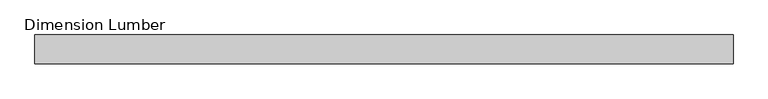
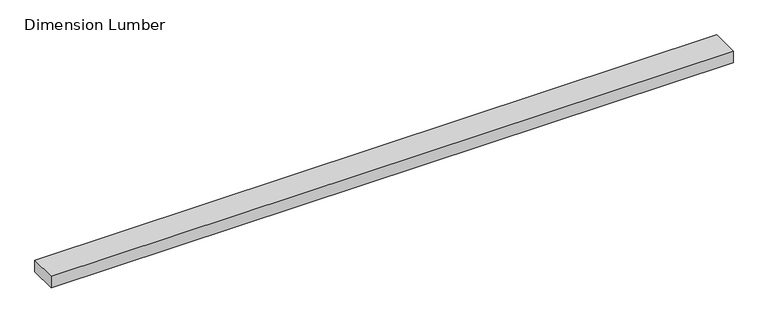
"""IFC4 building model written with IfcOpenShell, lengths in millimetres: beam geometry, Dimension Lumber : Top Supporting Lumbers."""

import ifcopenshell
import ifcopenshell.guid

model = None  # the IFC model being written
_history = None  # IfcOwnerHistory: only IFC2X3 demands one
_inside = {}  # id of a spatial element -> (the spatial element, [elements in it])
_under = {}  # id of a project, library or spatial element -> (it, [spatial elements below it])
_declared = {}  # id of a project -> (the project, [libraries it declares])
_typed = {}  # id of a type object -> (the type object, [elements of that type])
_made_of = {}  # id of a material, layer set ... -> (it, [elements and type objects made of it])


def new_model(schema):
    """Start an empty IFC model of exactly this schema.

    Asked for "IFC4X3", IfcOpenShell would pick the latest addendum, in which some entities
    have other attributes; the version numbers below select the first issue.
    IFC2X3 requires an IfcOwnerHistory on every rooted entity: one is made here for all.
    """
    global model, _history
    if schema == "IFC4X3":
        model = ifcopenshell.file(schema_version=(4, 3, 0, 0))
    else:
        model = ifcopenshell.file(schema=schema)
    _inside.clear()
    _under.clear()
    _declared.clear()
    _typed.clear()
    _made_of.clear()
    _history = None
    if model.schema == "IFC2X3":
        org = make("IfcOrganization", Name="unknown")
        user = make(
            "IfcPersonAndOrganization",
            ThePerson=make("IfcPerson", FamilyName="unknown"),
            TheOrganization=org,
        )
        app = make(
            "IfcApplication",
            ApplicationDeveloper=org,
            Version="unknown",
            ApplicationFullName="unknown",
            ApplicationIdentifier="unknown",
        )
        _history = make(
            "IfcOwnerHistory",
            OwningUser=user,
            OwningApplication=app,
            ChangeAction="ADDED",
            CreationDate=0,
        )
    return model


def make(cls, **values):
    """One entity of the class cls with the attributes given. An attribute that is None is left unset."""
    return model.create_entity(
        cls, **{name: value for name, value in values.items() if value is not None}
    )


def rooted(cls, **values):
    """An entity with a GlobalId (a new one), such as an element, a storey or a relation."""
    return make(cls, GlobalId=ifcopenshell.guid.new(), OwnerHistory=_history, **values)


def si_unit(unit_type, name, prefix=None):
    """IfcSIUnit, for example si_unit("LENGTHUNIT", "METRE", prefix="MILLI")."""
    return make("IfcSIUnit", UnitType=unit_type, Prefix=prefix, Name=name)


def assignment(units):
    """IfcUnitAssignment: the units of a project."""
    return None if units is None else make("IfcUnitAssignment", Units=units)


def point(xyz):
    """IfcCartesianPoint."""
    return None if xyz is None else make("IfcCartesianPoint", Coordinates=xyz)


def direction(xyz):
    """IfcDirection."""
    return None if xyz is None else make("IfcDirection", DirectionRatios=xyz)


def frame(location, z_axis=None, x_axis=None):
    """IfcAxis2Placement3D, a coordinate frame: its origin and axes. An axis left out is left unset."""
    return make(
        "IfcAxis2Placement3D",
        Location=point(location),
        Axis=direction(z_axis),
        RefDirection=direction(x_axis),
    )


def origin():
    """The frame at (0, 0, 0) with its axes left unset."""
    return frame((0.0, 0.0, 0.0))


def place(relative_to, where):
    """IfcLocalPlacement: puts the frame where relative to a parent placement (None: the world)."""
    return make(
        "IfcLocalPlacement", PlacementRelTo=relative_to, RelativePlacement=where
    )


def context(
    kind, dimensions, precision=None, world=None, true_north=None, identifier=None
):
    """IfcGeometricRepresentationContext, for example the 3D "Model" context."""
    return make(
        "IfcGeometricRepresentationContext",
        ContextIdentifier=identifier,
        ContextType=kind,
        CoordinateSpaceDimension=dimensions,
        Precision=precision,
        WorldCoordinateSystem=world,
        TrueNorth=true_north,
    )


def project(units=None, contexts=None):
    """IfcProject with its units and contexts."""
    return rooted(
        "IfcProject",
        Name="project",
        RepresentationContexts=contexts,
        UnitsInContext=assignment(units),
    )


def spatial(cls, under=None, at=None, **own):
    """A site, building, storey or space (cls), placed at a placement, below another one or the project."""
    s = rooted(cls, ObjectPlacement=at, **own)
    if under is not None:
        _under.setdefault(under.id(), (under, []))[1].append(s)
    return s


def polyline(points):
    """IfcPolyline through the points."""
    return make("IfcPolyline", Points=[point(p) for p in points])


def outline(outer, holes=None, kind="AREA"):
    """IfcArbitraryClosedProfileDef: a profile drawn as a closed curve; with holes, ...WithVoids."""
    if holes is None:
        return make("IfcArbitraryClosedProfileDef", ProfileType=kind, OuterCurve=outer)
    return make(
        "IfcArbitraryProfileDefWithVoids",
        ProfileType=kind,
        OuterCurve=outer,
        InnerCurves=holes,
    )


def extrude(swept, where, along, depth):
    """IfcExtrudedAreaSolid: the profile swept, set in the frame where, extruded along a direction by depth."""
    return make(
        "IfcExtrudedAreaSolid",
        SweptArea=swept,
        Position=where,
        ExtrudedDirection=direction(along),
        Depth=depth,
    )


def shape(context_of_items, identifier, shape_type, items):
    """IfcShapeRepresentation: the items that make up one representation, for example the "Body"."""
    return make(
        "IfcShapeRepresentation",
        ContextOfItems=context_of_items,
        RepresentationIdentifier=identifier,
        RepresentationType=shape_type,
        Items=items,
    )


def source(mapping_origin, context_of_items, identifier, shape_type, items):
    """IfcRepresentationMap: a shape defined once, which mapped items show again and again."""
    return make(
        "IfcRepresentationMap",
        MappingOrigin=mapping_origin,
        MappedRepresentation=shape(context_of_items, identifier, shape_type, items),
    )


def transform(
    local_origin,
    x_axis=None,
    y_axis=None,
    z_axis=None,
    scale=None,
    scale2=None,
    scale3=None,
    uniform=True,
):
    """IfcCartesianTransformationOperator3D, or its non-uniform kind. x_axis, y_axis, z_axis: its Axis1, 2, 3."""
    if uniform:
        return make(
            "IfcCartesianTransformationOperator3D",
            Axis1=direction(x_axis),
            Axis2=direction(y_axis),
            LocalOrigin=point(local_origin),
            Scale=scale,
            Axis3=direction(z_axis),
        )
    return make(
        "IfcCartesianTransformationOperator3DnonUniform",
        Axis1=direction(x_axis),
        Axis2=direction(y_axis),
        LocalOrigin=point(local_origin),
        Scale=scale,
        Axis3=direction(z_axis),
        Scale2=scale2,
        Scale3=scale3,
    )


def mapped(mapping_source, mapping_target):
    """IfcMappedItem: shows the shape of a source again, moved by a transform."""
    return make(
        "IfcMappedItem", MappingSource=mapping_source, MappingTarget=mapping_target
    )


def made_of(thing, what):
    """Note that an element or type object is made of a material, layer set ...; save() writes the relation."""
    if what is not None:
        _made_of.setdefault(what.id(), (what, []))[1].append(thing)
    return thing


def element(
    cls,
    number,
    at=None,
    inside=None,
    cuts=None,
    type_object=None,
    material=None,
    context=None,
    identifier="Body",
    shape_type=None,
    held_by="IfcProductDefinitionShape",
    body=None,
    shapes=None,
    **own,
):
    """One element of the class cls, such as IfcWall. Its Tag is "e" and its number.

    at: its placement. inside: the storey or other place that contains it. cuts: it is an
    opening in that element (IfcRelVoidsElement). A single representation is given by context,
    identifier, shape_type and body (its items); several are given by shapes. held_by: the class
    of the entity that holds the representations. save() writes the other relations.
    """
    e = rooted(cls, Tag="e%d" % number, ObjectPlacement=at, **own)
    if body is not None:
        shapes = [shape(context, identifier, shape_type, body)]
    if shapes is not None:
        e.Representation = make(held_by, Representations=shapes)
    if inside is not None:
        _inside.setdefault(inside.id(), (inside, []))[1].append(e)
    if cuts is not None:
        rooted(
            "IfcRelVoidsElement", RelatingBuildingElement=cuts, RelatedOpeningElement=e
        )
    if type_object is not None:
        _typed.setdefault(type_object.id(), (type_object, []))[1].append(e)
    return made_of(e, material)


def aggregate(whole, parts):
    """IfcRelAggregates: a whole, such as a stair, and the parts it consists of."""
    return rooted("IfcRelAggregates", RelatingObject=whole, RelatedObjects=parts)


def save(model, path):
    """Write the relations noted so far, then the file.

    IfcRelAggregates (storeys below a building ...), IfcRelContainedInSpatialStructure (elements
    in a storey), IfcRelDefinesByType, IfcRelAssociatesMaterial and IfcRelDeclares: one each for
    every whole, place, type object, material and project.
    """
    for whole, parts in _under.values():
        aggregate(whole, parts)
    for where, things in _inside.values():
        rooted(
            "IfcRelContainedInSpatialStructure",
            RelatedElements=things,
            RelatingStructure=where,
        )
    for kind, things in _typed.values():
        rooted("IfcRelDefinesByType", RelatedObjects=things, RelatingType=kind)
    for what, things in _made_of.values():
        rooted("IfcRelAssociatesMaterial", RelatedObjects=things, RelatingMaterial=what)
    for by, libraries in _declared.values():
        rooted("IfcRelDeclares", RelatingContext=by, RelatedDefinitions=libraries)
    model.write(path)


def dimension_lumber_386be09e(model_context):
    return source(origin(), model_context, "Body", "SweptSolid", [
        extrude(outline(polyline([(1073.15, 44.45), (1073.15, -44.45), (-1073.15, -44.45), (-1073.15, 44.45), (1073.15, 44.45)])), frame((0.0, 0.0, -19.05), z_axis=(0.0, 0.0, 1.0), x_axis=(1.0, 0.0, 0.0)), (0.0, 0.0, 1.0), 38.1),
    ])


if __name__ == "__main__":
    model = new_model("IFC4")
    model_context = context("Model", 3, world=origin())
    ifc_project = project(units=[si_unit("LENGTHUNIT", "METRE", prefix="MILLI")], contexts=[model_context])
    site = spatial("IfcSite", under=ifc_project)
    building = spatial("IfcBuilding", under=site)
    placement = place(None, origin())
    dimension_lumber_shape = dimension_lumber_386be09e(model_context)
    element("IfcBeam", 1, ObjectType="Dimension Lumber : Top Supporting Lumbers", at=placement, inside=building, context=model_context, shape_type="MappedRepresentation", body=[
        mapped(dimension_lumber_shape, transform((0.0, 0.0, 0.0), x_axis=(1.0, 0.0, 0.0), y_axis=(0.0, 1.0, 0.0), z_axis=(0.0, 0.0, 1.0))),
    ])
    save(model, "model.ifc")

# Revit data of these elements
# Type "Dimension Lumber : Top Supporting Lumbers"
#   Assembly Code = "B10"
#   A = 0.0364583 SF
#   Length [instance default] = 5' - 0"
#   b = 0' - 3 1/2"
#   d = 0' - 1 1/2"
#   Structural Material [instance default] = Softwood, Lumber
# Element 1 (IfcBeam, "Dimension Lumber : Top Supporting Lumbers")
#   Structural Material = Douglas Fir #2
#   Materials on its faces: "Douglas Fir #2"
# Materials
#   "Softwood, Lumber": class "Wood", colour RGB 223 192 134, transparency 0, Description = "Pinus Echinata", Cost = 0
#   "Douglas Fir #2": class "Wood", colour RGB 223 192 134, transparency 0, Description = "Pinus Echinata", Cost = 0
